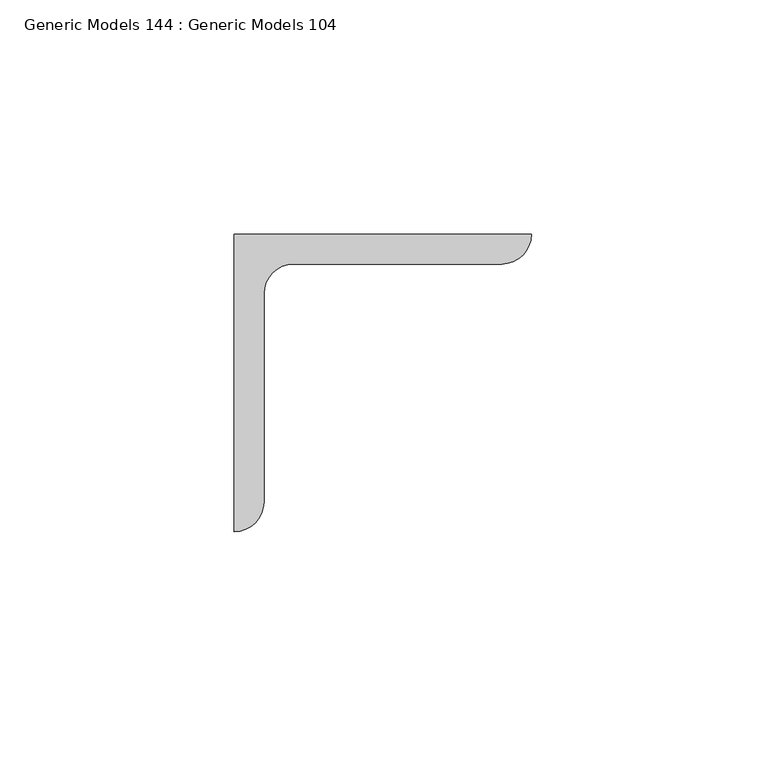
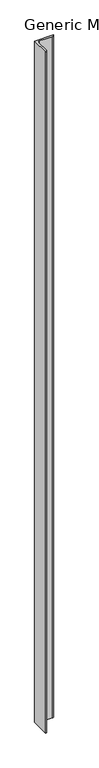
"""IFC4 building model written with IfcOpenShell, lengths in millimetres: proxy geometry, Generic Models 144 : Generic Models 104."""

from ifc_helpers import new_model, si_unit, point, frame, frame_2d, origin, place, context, project, spatial, polyline, circle_curve, trimmed, segment, composite_curve, outline, extrude, source, transform, mapped, element, save


def generic_models_144_generic_models_104_8f00bb07(model_context):
    return source(origin(), model_context, "Body", "SweptSolid", [
        extrude(outline(composite_curve([segment(polyline([(34428.1090778, 41071.1196612), (34491.6090778, 41071.1196612)]), True, "CONTINUOUS"), segment(trimmed(circle_curve(frame_2d((34485.2590778, 41071.1196612)), 6.35), [point((34491.6090778, 41071.1196612))], [point((34485.2590778, 41064.7696612))], False, "CARTESIAN"), True, "CONTINUOUS"), segment(polyline([(34485.2590778, 41064.7696612), (34440.8090778, 41064.7696612)]), True, "CONTINUOUS"), segment(trimmed(circle_curve(frame_2d((34440.8090778, 41058.4196612)), 6.35), [point((34440.8090778, 41064.7696612))], [point((34434.4590778, 41058.4196612))], True, "CARTESIAN"), True, "CONTINUOUS"), segment(polyline([(34434.4590778, 41058.4196612), (34434.4590778, 41013.9696612)]), True, "CONTINUOUS"), segment(trimmed(circle_curve(frame_2d((34428.1090778, 41013.9696612)), 6.35), [point((34434.4590778, 41013.9696612))], [point((34428.1090778, 41007.6196612))], False, "CARTESIAN"), True, "CONTINUOUS"), segment(polyline([(34428.1090778, 41007.6196612), (34428.1090778, 41071.1196612)]), True, "CONTINUOUS")], self_intersect=False)), frame((0.0, 0.0, 266407.9), z_axis=(0.0, 0.0, 1.0), x_axis=(1.0, 0.0, 0.0)), (0.0, 0.0, 1.0), 2432.1044757),
    ])


if __name__ == "__main__":
    model = new_model("IFC4")
    model_context = context("Model", 3, world=origin())
    ifc_project = project(units=[si_unit("LENGTHUNIT", "METRE", prefix="MILLI")], contexts=[model_context])
    site = spatial("IfcSite", under=ifc_project)
    building = spatial("IfcBuilding", under=site)
    placement = place(None, origin())
    generic_models_144_generic_models_104_shape = generic_models_144_generic_models_104_8f00bb07(model_context)
    element("IfcBuildingElementProxy", 1, Name="Generic Models 144 : Generic Models 104", ObjectType="Generic Models 144 : Generic Models 104", at=placement, inside=building, context=model_context, shape_type="MappedRepresentation", body=[
        mapped(generic_models_144_generic_models_104_shape, transform((0.0, 0.0, 0.0), x_axis=(1.0, 0.0, 0.0), y_axis=(0.0, 1.0, 0.0), z_axis=(0.0, 0.0, 1.0))),
    ])
    save(model, "model.ifc")

# Revit data of these elements
# Element 1 (IfcBuildingElementProxy, "Generic Models 144 : Generic Models 104")
#   Materials on its faces: "(2) BACK/BACK GALVANIZED ANGLES (2) L2 1/2 X 2 1/2 X 1/4\")"
# Materials
#   "(2) BACK/BACK GALVANIZED ANGLES (2) L2 1/2 X 2 1/2 X 1/4\")": class "Unassigned", colour RGB 211 211 211, transparency 0, Cost = 0
